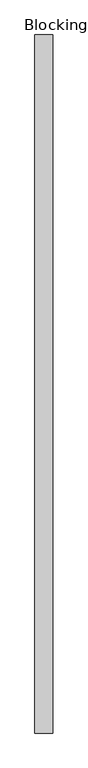
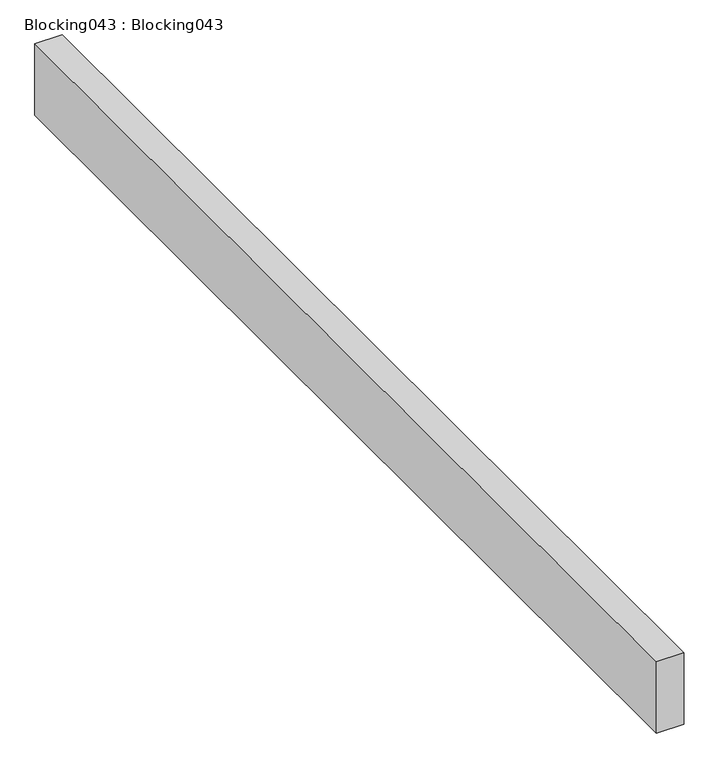
"""IFC4 building model written with IfcOpenShell, lengths in millimetres: proxy geometry, Blocking043 : Blocking043."""

import ifcopenshell
import ifcopenshell.guid

model = None  # the IFC model being written
_history = None  # IfcOwnerHistory: only IFC2X3 demands one
_inside = {}  # id of a spatial element -> (the spatial element, [elements in it])
_under = {}  # id of a project, library or spatial element -> (it, [spatial elements below it])
_declared = {}  # id of a project -> (the project, [libraries it declares])
_typed = {}  # id of a type object -> (the type object, [elements of that type])
_made_of = {}  # id of a material, layer set ... -> (it, [elements and type objects made of it])


def new_model(schema):
    """Start an empty IFC model of exactly this schema.

    Asked for "IFC4X3", IfcOpenShell would pick the latest addendum, in which some entities
    have other attributes; the version numbers below select the first issue.
    IFC2X3 requires an IfcOwnerHistory on every rooted entity: one is made here for all.
    """
    global model, _history
    if schema == "IFC4X3":
        model = ifcopenshell.file(schema_version=(4, 3, 0, 0))
    else:
        model = ifcopenshell.file(schema=schema)
    _inside.clear()
    _under.clear()
    _declared.clear()
    _typed.clear()
    _made_of.clear()
    _history = None
    if model.schema == "IFC2X3":
        org = make("IfcOrganization", Name="unknown")
        user = make(
            "IfcPersonAndOrganization",
            ThePerson=make("IfcPerson", FamilyName="unknown"),
            TheOrganization=org,
        )
        app = make(
            "IfcApplication",
            ApplicationDeveloper=org,
            Version="unknown",
            ApplicationFullName="unknown",
            ApplicationIdentifier="unknown",
        )
        _history = make(
            "IfcOwnerHistory",
            OwningUser=user,
            OwningApplication=app,
            ChangeAction="ADDED",
            CreationDate=0,
        )
    return model


def make(cls, **values):
    """One entity of the class cls with the attributes given. An attribute that is None is left unset."""
    return model.create_entity(
        cls, **{name: value for name, value in values.items() if value is not None}
    )


def rooted(cls, **values):
    """An entity with a GlobalId (a new one), such as an element, a storey or a relation."""
    return make(cls, GlobalId=ifcopenshell.guid.new(), OwnerHistory=_history, **values)


def si_unit(unit_type, name, prefix=None):
    """IfcSIUnit, for example si_unit("LENGTHUNIT", "METRE", prefix="MILLI")."""
    return make("IfcSIUnit", UnitType=unit_type, Prefix=prefix, Name=name)


def assignment(units):
    """IfcUnitAssignment: the units of a project."""
    return None if units is None else make("IfcUnitAssignment", Units=units)


def point(xyz):
    """IfcCartesianPoint."""
    return None if xyz is None else make("IfcCartesianPoint", Coordinates=xyz)


def direction(xyz):
    """IfcDirection."""
    return None if xyz is None else make("IfcDirection", DirectionRatios=xyz)


def frame(location, z_axis=None, x_axis=None):
    """IfcAxis2Placement3D, a coordinate frame: its origin and axes. An axis left out is left unset."""
    return make(
        "IfcAxis2Placement3D",
        Location=point(location),
        Axis=direction(z_axis),
        RefDirection=direction(x_axis),
    )


def origin():
    """The frame at (0, 0, 0) with its axes left unset."""
    return frame((0.0, 0.0, 0.0))


def place(relative_to, where):
    """IfcLocalPlacement: puts the frame where relative to a parent placement (None: the world)."""
    return make(
        "IfcLocalPlacement", PlacementRelTo=relative_to, RelativePlacement=where
    )


def context(
    kind, dimensions, precision=None, world=None, true_north=None, identifier=None
):
    """IfcGeometricRepresentationContext, for example the 3D "Model" context."""
    return make(
        "IfcGeometricRepresentationContext",
        ContextIdentifier=identifier,
        ContextType=kind,
        CoordinateSpaceDimension=dimensions,
        Precision=precision,
        WorldCoordinateSystem=world,
        TrueNorth=true_north,
    )


def project(units=None, contexts=None):
    """IfcProject with its units and contexts."""
    return rooted(
        "IfcProject",
        Name="project",
        RepresentationContexts=contexts,
        UnitsInContext=assignment(units),
    )


def spatial(cls, under=None, at=None, **own):
    """A site, building, storey or space (cls), placed at a placement, below another one or the project."""
    s = rooted(cls, ObjectPlacement=at, **own)
    if under is not None:
        _under.setdefault(under.id(), (under, []))[1].append(s)
    return s


def polyline(points):
    """IfcPolyline through the points."""
    return make("IfcPolyline", Points=[point(p) for p in points])


def outline(outer, holes=None, kind="AREA"):
    """IfcArbitraryClosedProfileDef: a profile drawn as a closed curve; with holes, ...WithVoids."""
    if holes is None:
        return make("IfcArbitraryClosedProfileDef", ProfileType=kind, OuterCurve=outer)
    return make(
        "IfcArbitraryProfileDefWithVoids",
        ProfileType=kind,
        OuterCurve=outer,
        InnerCurves=holes,
    )


def extrude(swept, where, along, depth):
    """IfcExtrudedAreaSolid: the profile swept, set in the frame where, extruded along a direction by depth."""
    return make(
        "IfcExtrudedAreaSolid",
        SweptArea=swept,
        Position=where,
        ExtrudedDirection=direction(along),
        Depth=depth,
    )


def shape(context_of_items, identifier, shape_type, items):
    """IfcShapeRepresentation: the items that make up one representation, for example the "Body"."""
    return make(
        "IfcShapeRepresentation",
        ContextOfItems=context_of_items,
        RepresentationIdentifier=identifier,
        RepresentationType=shape_type,
        Items=items,
    )


def source(mapping_origin, context_of_items, identifier, shape_type, items):
    """IfcRepresentationMap: a shape defined once, which mapped items show again and again."""
    return make(
        "IfcRepresentationMap",
        MappingOrigin=mapping_origin,
        MappedRepresentation=shape(context_of_items, identifier, shape_type, items),
    )


def transform(
    local_origin,
    x_axis=None,
    y_axis=None,
    z_axis=None,
    scale=None,
    scale2=None,
    scale3=None,
    uniform=True,
):
    """IfcCartesianTransformationOperator3D, or its non-uniform kind. x_axis, y_axis, z_axis: its Axis1, 2, 3."""
    if uniform:
        return make(
            "IfcCartesianTransformationOperator3D",
            Axis1=direction(x_axis),
            Axis2=direction(y_axis),
            LocalOrigin=point(local_origin),
            Scale=scale,
            Axis3=direction(z_axis),
        )
    return make(
        "IfcCartesianTransformationOperator3DnonUniform",
        Axis1=direction(x_axis),
        Axis2=direction(y_axis),
        LocalOrigin=point(local_origin),
        Scale=scale,
        Axis3=direction(z_axis),
        Scale2=scale2,
        Scale3=scale3,
    )


def mapped(mapping_source, mapping_target):
    """IfcMappedItem: shows the shape of a source again, moved by a transform."""
    return make(
        "IfcMappedItem", MappingSource=mapping_source, MappingTarget=mapping_target
    )


def made_of(thing, what):
    """Note that an element or type object is made of a material, layer set ...; save() writes the relation."""
    if what is not None:
        _made_of.setdefault(what.id(), (what, []))[1].append(thing)
    return thing


def element(
    cls,
    number,
    at=None,
    inside=None,
    cuts=None,
    type_object=None,
    material=None,
    context=None,
    identifier="Body",
    shape_type=None,
    held_by="IfcProductDefinitionShape",
    body=None,
    shapes=None,
    **own,
):
    """One element of the class cls, such as IfcWall. Its Tag is "e" and its number.

    at: its placement. inside: the storey or other place that contains it. cuts: it is an
    opening in that element (IfcRelVoidsElement). A single representation is given by context,
    identifier, shape_type and body (its items); several are given by shapes. held_by: the class
    of the entity that holds the representations. save() writes the other relations.
    """
    e = rooted(cls, Tag="e%d" % number, ObjectPlacement=at, **own)
    if body is not None:
        shapes = [shape(context, identifier, shape_type, body)]
    if shapes is not None:
        e.Representation = make(held_by, Representations=shapes)
    if inside is not None:
        _inside.setdefault(inside.id(), (inside, []))[1].append(e)
    if cuts is not None:
        rooted(
            "IfcRelVoidsElement", RelatingBuildingElement=cuts, RelatedOpeningElement=e
        )
    if type_object is not None:
        _typed.setdefault(type_object.id(), (type_object, []))[1].append(e)
    return made_of(e, material)


def aggregate(whole, parts):
    """IfcRelAggregates: a whole, such as a stair, and the parts it consists of."""
    return rooted("IfcRelAggregates", RelatingObject=whole, RelatedObjects=parts)


def save(model, path):
    """Write the relations noted so far, then the file.

    IfcRelAggregates (storeys below a building ...), IfcRelContainedInSpatialStructure (elements
    in a storey), IfcRelDefinesByType, IfcRelAssociatesMaterial and IfcRelDeclares: one each for
    every whole, place, type object, material and project.
    """
    for whole, parts in _under.values():
        aggregate(whole, parts)
    for where, things in _inside.values():
        rooted(
            "IfcRelContainedInSpatialStructure",
            RelatedElements=things,
            RelatingStructure=where,
        )
    for kind, things in _typed.values():
        rooted("IfcRelDefinesByType", RelatedObjects=things, RelatingType=kind)
    for what, things in _made_of.values():
        rooted("IfcRelAssociatesMaterial", RelatedObjects=things, RelatingMaterial=what)
    for by, libraries in _declared.values():
        rooted("IfcRelDeclares", RelatingContext=by, RelatedDefinitions=libraries)
    model.write(path)


def blocking043_blocking043_a51c543b(model_context):
    return source(origin(), model_context, "Body", "SweptSolid", [
        extrude(outline(polyline([(-2694.3737014, -1052.8908936), (-2745.1737014, -1052.8908936), (-2745.1737014, 947.1091064), (-2694.3737014, 947.1091064), (-2694.3737014, -1052.8908936)])), frame((0.0, 0.0, 39579.2960083), z_axis=(0.0, 0.0, 1.0), x_axis=(1.0, 0.0, 0.0)), (0.0, 0.0, 1.0), 139.7),
    ])


if __name__ == "__main__":
    model = new_model("IFC4")
    model_context = context("Model", 3, world=origin())
    ifc_project = project(units=[si_unit("LENGTHUNIT", "METRE", prefix="MILLI")], contexts=[model_context])
    site = spatial("IfcSite", under=ifc_project)
    building = spatial("IfcBuilding", under=site)
    placement = place(None, origin())
    blocking043_blocking043_shape = blocking043_blocking043_a51c543b(model_context)
    element("IfcBuildingElementProxy", 1, Name="Blocking043 : Blocking043", ObjectType="Blocking043 : Blocking043", at=placement, inside=building, context=model_context, shape_type="MappedRepresentation", body=[
        mapped(blocking043_blocking043_shape, transform((0.0, 0.0, 0.0), x_axis=(1.0, 0.0, 0.0), y_axis=(0.0, 1.0, 0.0), z_axis=(0.0, 0.0, 1.0))),
    ])
    save(model, "model.ifc")

# Revit data of these elements
# Type "Blocking043 : Blocking043"
#   NameOverride = "Blocking043"
# Element 1 (IfcBuildingElementProxy, "Blocking043 : Blocking043")
#   Materials on its faces: "WOOD BLOCKING AS REQUIRED"
# Materials
#   "WOOD BLOCKING AS REQUIRED": class "Unassigned", colour RGB 166 124 85, transparency 0, Cost = 0
